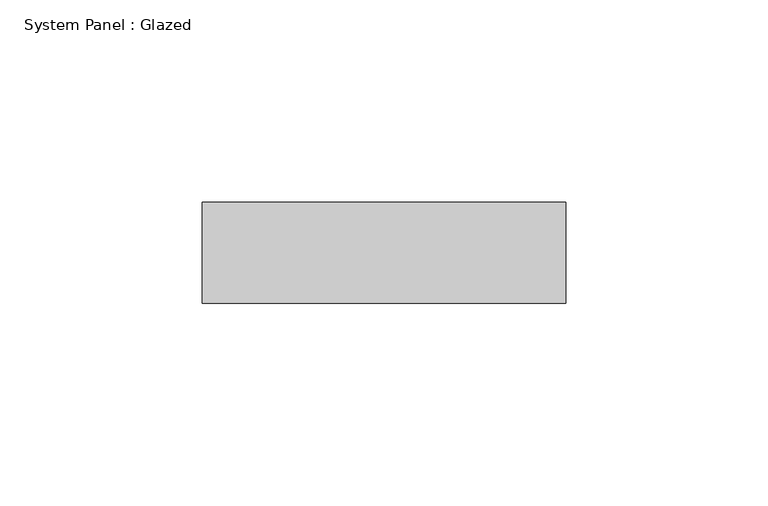
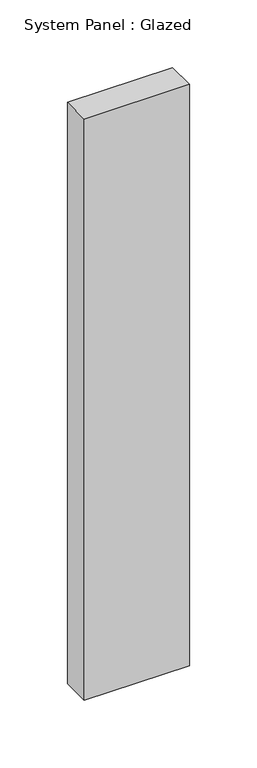
"""IFC4 building model written with IfcOpenShell, lengths in millimetres: plate geometry, System Panel : Glazed."""

from ifc_helpers import new_model, si_unit, origin, origin_with_axes, place, context, project, spatial, polyline, outline, extrude, source, transform, mapped, element, save


def system_panel_glazed_1504e954(model_context):
    return source(origin(), model_context, "Body", "SweptSolid", [
        extrude(outline(polyline([(44.9999998, 24.5), (-44.9999998, 24.5), (-44.9999998, 49.5), (44.9999998, 49.5), (44.9999998, 24.5)])), origin_with_axes(), (0.0, 0.0, 1.0), 525.0),
    ])


if __name__ == "__main__":
    model = new_model("IFC4")
    model_context = context("Model", 3, world=origin())
    ifc_project = project(units=[si_unit("LENGTHUNIT", "METRE", prefix="MILLI")], contexts=[model_context])
    site = spatial("IfcSite", under=ifc_project)
    building = spatial("IfcBuilding", under=site)
    placement = place(None, origin())
    system_panel_glazed_shape = system_panel_glazed_1504e954(model_context)
    element("IfcPlate", 1, ObjectType="System Panel : Glazed", at=placement, inside=building, context=model_context, shape_type="MappedRepresentation", body=[
        mapped(system_panel_glazed_shape, transform((0.0, 0.0, 0.0), x_axis=(1.0, 0.0, 0.0), y_axis=(0.0, 1.0, 0.0), z_axis=(0.0, 0.0, 1.0))),
    ])
    save(model, "model.ifc")

# Revit data of these elements
# Element 1 (IfcPlate, "System Panel : Glazed")
#   Materials on its faces: "Glass"
# Materials
#   "Glass": class "Glass", colour RGB 218 227 224, transparency 0.85, Description = "Soda Lime Glass", Cost = 0
